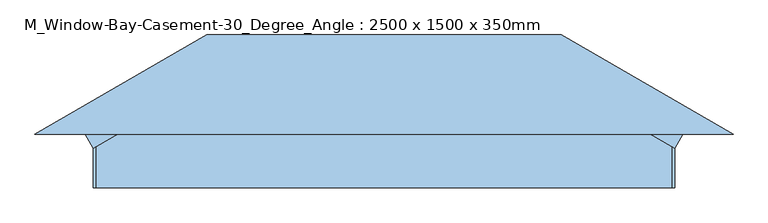
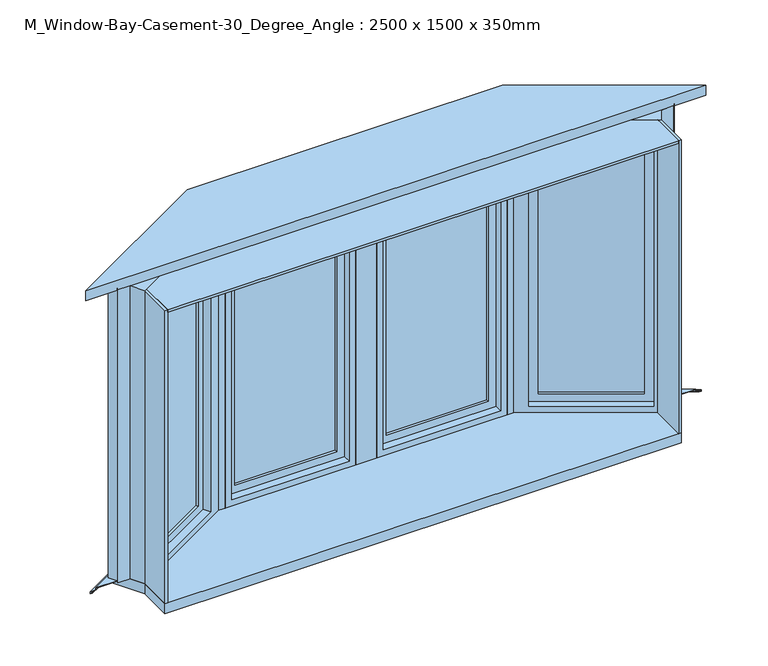
"""IFC4 building model written with IfcOpenShell, lengths in millimetres: window geometry, M_Window-Bay-Casement-30_Degree_Angle : 2500 x 1500 x 350mm."""

from ifc_helpers import new_model, si_unit, frame, origin, place, context, project, spatial, polyline, outline, extrude, faceted_brep, source, transform, mapped, element, save


def m_window_bay_casement_30_degree_angle_2500_x_1500_x_350mm_0714d089(model_context):
    return source(origin(), model_context, "Body", "SolidModel", [
        extrude(outline(polyline([(1224.4331255, 149.925), (1221.2581255, 144.4257387), (835.0107955, 367.4257387), (838.1857955, 372.925), (1224.4331255, 149.925)])), frame((0.0, 0.0, 720.65), z_axis=(0.0, 0.0, 1.0), x_axis=(1.0, 0.0, 0.0)), (0.0, 0.0, 1.0), 1360.3),
        extrude(outline(polyline([(1218.0831255, 138.9264774), (1214.9081255, 133.4272161), (828.6607955, 356.4272161), (831.8357955, 361.9264774), (1218.0831255, 138.9264774)])), frame((0.0, 0.0, 720.65), z_axis=(0.0, 0.0, 1.0), x_axis=(1.0, 0.0, 0.0)), (0.0, 0.0, 1.0), 1360.3),
        extrude(outline(polyline([(1417.45, 57.1500001), (1417.45, -503.15), (-57.15, -503.15), (-57.15, 57.1500001), (1417.45, 57.1500001)]), holes=[polyline([(1360.3, -445.9999999), (1360.3, 0.0), (0.0, 0.0), (0.0, -445.9999999), (1360.3, -445.9999999)])]), frame((1208.5581255, 122.4286934, 720.65), z_axis=(0.49999999999999967, 0.8660254037844388, 0.0), x_axis=(0.0, 0.0, 1.0)), (0.0, 0.0, 1.0), 44.45),
        faceted_brep([(714.9835794, 363.4, 2150.8), (1250.0, 54.5081255, 2150.8), (1284.925, 115.0, 2150.8), (1344.7940905, 115.0, 2150.8), (1344.7940905, 117.0963066, 2150.8), (742.2072174, 465.0, 2150.8), (1258.0514774, 93.8536934, 2138.1), (772.8174436, 374.0036934, 2138.1), (804.5674436, 428.9963066, 2138.1), (1289.8014774, 148.8463066, 2138.1), (1222.5036934, 70.3831255, 2119.05), (770.2652276, 331.4831255, 2119.05), (789.3152276, 364.4786934, 2119.05), (1241.5536934, 103.3786934, 2119.05), (772.8174436, 374.0036934, 663.5), (804.5674436, 428.9963066, 663.5), (770.2652276, 331.4831255, 682.55), (789.3152276, 364.4786934, 682.55), (742.2072174, 465.0, 650.8), (1344.7940905, 117.0963066, 650.8), (1344.7940905, 115.0, 650.8), (1284.925, 115.0, 650.8), (1250.0, 54.5081255, 650.8), (714.9835794, 363.4, 650.8), (1258.0514774, 93.8536934, 663.5), (1289.8014774, 148.8463066, 663.5), (1222.5036934, 70.3831255, 682.55), (1241.5536934, 103.3786934, 682.55)], [[[0, 1, 2, 3, 4, 5]], [[6, 7, 8, 9]], [[10, 11, 12, 13]], [[7, 14, 15, 8]], [[11, 16, 17, 12]], [[18, 19, 20, 21, 22, 23]], [[14, 24, 25, 15]], [[16, 26, 27, 17]], [[22, 21, 2, 1]], [[4, 19, 18, 5], [8, 15, 25, 9]], [[9, 25, 24, 6]], [[6, 24, 14, 7], [12, 17, 27, 13]], [[13, 27, 26, 10]], [[1, 0, 23, 22], [10, 26, 16, 11]], [[5, 18, 23, 0]], [[2, 21, 20, 3]], [[3, 20, 19, 4]]]),
        extrude(outline(polyline([(-1224.4331255, 149.925), (-838.1857955, 372.925), (-835.0107955, 367.4257387), (-1221.2581255, 144.4257387), (-1224.4331255, 149.925)])), frame((0.0, 0.0, 720.65), z_axis=(0.0, 0.0, 1.0), x_axis=(1.0, 0.0, 0.0)), (0.0, 0.0, 1.0), 1360.3),
        extrude(outline(polyline([(-1218.0831255, 138.9264774), (-831.8357955, 361.9264774), (-828.6607955, 356.4272161), (-1214.9081255, 133.4272161), (-1218.0831255, 138.9264774)])), frame((0.0, 0.0, 720.65), z_axis=(0.0, 0.0, 1.0), x_axis=(1.0, 0.0, 0.0)), (0.0, 0.0, 1.0), 1360.3),
        extrude(outline(polyline([(1417.45, -57.1500001), (-57.15, -57.1500001), (-57.15, 503.15), (1417.45, 503.15), (1417.45, -57.1500001)]), holes=[polyline([(1360.3, 445.9999999), (0.0, 445.9999999), (0.0, 0.0), (1360.3, 0.0), (1360.3, 445.9999999)])]), frame((-1208.5581255, 122.4286934, 720.65), z_axis=(-0.49999999999999967, 0.8660254037844388, 0.0), x_axis=(0.0, 0.0, 1.0)), (0.0, 0.0, 1.0), 44.45),
        faceted_brep([(-714.9835794, 363.4, 2150.8), (-742.2072174, 465.0, 2150.8), (-1344.7940905, 117.0963066, 2150.8), (-1344.7940905, 115.0, 2150.8), (-1284.925, 115.0, 2150.8), (-1250.0, 54.5081255, 2150.8), (-1258.0514774, 93.8536934, 2138.1), (-1289.8014774, 148.8463066, 2138.1), (-804.5674436, 428.9963066, 2138.1), (-772.8174436, 374.0036934, 2138.1), (-1222.5036934, 70.3831255, 2119.05), (-1241.5536934, 103.3786934, 2119.05), (-789.3152276, 364.4786934, 2119.05), (-770.2652276, 331.4831255, 2119.05), (-804.5674436, 428.9963066, 663.5), (-772.8174436, 374.0036934, 663.5), (-789.3152276, 364.4786934, 682.55), (-770.2652276, 331.4831255, 682.55), (-742.2072174, 465.0, 650.8), (-714.9835794, 363.4, 650.8), (-1250.0, 54.5081255, 650.8), (-1284.925, 115.0, 650.8), (-1344.7940905, 115.0, 650.8), (-1344.7940905, 117.0963066, 650.8), (-1289.8014774, 148.8463066, 663.5), (-1258.0514774, 93.8536934, 663.5), (-1241.5536934, 103.3786934, 682.55), (-1222.5036934, 70.3831255, 682.55)], [[[0, 1, 2, 3, 4, 5]], [[6, 7, 8, 9]], [[10, 11, 12, 13]], [[9, 8, 14, 15]], [[13, 12, 16, 17]], [[18, 19, 20, 21, 22, 23]], [[15, 14, 24, 25]], [[17, 16, 26, 27]], [[20, 5, 4, 21]], [[2, 1, 18, 23], [8, 7, 24, 14]], [[7, 6, 25, 24]], [[6, 9, 15, 25], [12, 11, 26, 16]], [[11, 10, 27, 26]], [[5, 20, 19, 0], [10, 13, 17, 27]], [[1, 0, 19, 18]], [[4, 3, 22, 21]], [[3, 2, 23, 22]]]),
        faceted_brep([(-755.844462, 515.8, 660.4), (-755.844462, 515.8, 653.0697935), (755.844462, 515.8, 653.0697935), (755.844462, 515.8, 660.4), (-742.232643, 465.0, 663.1486341), (-742.232643, 465.0, 660.4), (742.232643, 465.0, 660.4), (742.232643, 465.0, 663.1486341), (-756.218787, 517.197, 654.4483503), (-756.218787, 517.197, 663.1486341), (756.218787, 517.197, 663.1486341), (756.218787, 517.197, 654.4483503), (759.6217417, 529.897, 652.2089977), (-759.6217417, 529.897, 652.2089977), (759.6217417, 529.897, 643.2668038), (-759.6217417, 529.897, 643.2668038), (-758.5600199, 525.9346, 644.7270038), (-758.5600199, 525.9346, 643.2668038), (758.5600199, 525.9346, 643.2668038), (758.5600199, 525.9346, 644.7270038), (-759.1929694, 528.2968, 650.8662705), (-759.1929694, 528.2968, 644.7270038), (759.1929694, 528.2968, 644.7270038), (759.1929694, 528.2968, 650.8662705), (-1450.0504256, 115.0, 660.4), (-1450.0504256, 115.0, 653.0697935), (1450.0504256, 115.0, 660.4), (1348.4504256, 115.0, 660.4), (-1348.4504256, 115.0, 660.4), (-1348.4504256, 115.0, 663.1486341), (1348.4504256, 115.0, 663.1486341), (1452.8444256, 115.0, 663.1486341), (-1452.8444256, 115.0, 663.1486341), (-1452.8444256, 115.0, 654.4483503), (-1478.2444256, 115.0, 652.2089977), (-1478.2444256, 115.0, 643.2668038), (1478.2444256, 115.0, 643.2668038), (1470.3196257, 115.0, 643.2668038), (-1470.3196257, 115.0, 643.2668038), (-1470.3196257, 115.0, 644.7270038), (1470.3196257, 115.0, 644.7270038), (1475.0440256, 115.0, 644.7270038), (-1475.0440256, 115.0, 644.7270038), (-1475.0440256, 115.0, 650.8662705), (1450.0504256, 115.0, 653.0697935), (1452.8444256, 115.0, 654.4483503), (1478.2444256, 115.0, 652.2089977), (1475.0440256, 115.0, 650.8662705)], [[[0, 1, 2, 3]], [[4, 5, 6, 7]], [[8, 9, 10, 11]], [[8, 11, 12, 13]], [[13, 12, 14, 15]], [[16, 17, 18, 19]], [[20, 21, 22, 23]], [[2, 1, 20, 23]], [[1, 0, 24, 25]], [[0, 3, 26, 27, 6, 5, 28, 24]], [[5, 4, 29, 28]], [[4, 7, 30, 31, 10, 9, 32, 29]], [[9, 8, 33, 32]], [[8, 13, 34, 33]], [[13, 15, 35, 34]], [[15, 14, 36, 37, 18, 17, 38, 35]], [[17, 16, 39, 38]], [[16, 19, 40, 41, 22, 21, 42, 39]], [[21, 20, 43, 42]], [[20, 1, 25, 43]], [[3, 2, 44, 26]], [[7, 6, 27, 30]], [[11, 10, 31, 45]], [[12, 11, 45, 46]], [[14, 12, 46, 36]], [[19, 18, 37, 40]], [[23, 22, 41, 47]], [[2, 23, 47, 44]], [[25, 24, 28, 29, 32, 33, 34, 35, 38, 39, 42, 43]], [[27, 26, 44, 47, 41, 40, 37, 36, 46, 45, 31, 30]]]),
        extrude(outline(polyline([(-1320.9541191, 130.875), (-1348.4504256, 115.0), (-1370.6754256, 153.4948292), (-1343.1791191, 169.3698292), (-1320.9541191, 130.875)])), frame((0.0, 0.0, 663.1486341), z_axis=(0.0, 0.0, 1.0), x_axis=(1.0, 0.0, 0.0)), (0.0, 0.0, 1.0), 1497.2513659),
        extrude(outline(polyline([(1320.9541191, 130.875), (1343.1791191, 169.3698292), (1370.6754256, 153.4948292), (1348.4504256, 115.0), (1320.9541191, 130.875)])), frame((0.0, 0.0, 663.1486341), z_axis=(0.0, 0.0, 1.0), x_axis=(1.0, 0.0, 0.0)), (0.0, 0.0, 1.0), 1497.2513659),
        extrude(outline(polyline([(-714.9835794, 363.4), (714.9835794, 363.4), (1237.3, 61.840474), (1237.3, -115.0), (-1237.3, -115.0), (-1237.3, 61.840474), (-714.9835794, 363.4)])), frame((0.0, 0.0, 2138.1), z_axis=(0.0, 0.0, 1.0), x_axis=(1.0, 0.0, 0.0)), (0.0, 0.0, 1.0), 12.7),
        extrude(outline(polyline([(-1250.0, -115.0), (-1250.0, 54.5081255), (-1237.3, 61.840474), (-1237.3, -115.0), (-1250.0, -115.0)])), frame((0.0, 0.0, 650.8), z_axis=(0.0, 0.0, 1.0), x_axis=(1.0, 0.0, 0.0)), (0.0, 0.0, 1.0), 1500.0),
        extrude(outline(polyline([(1250.0, -115.0), (1237.3, -115.0), (1237.3, 61.840474), (1250.0, 54.5081256), (1250.0, -115.0)])), frame((0.0, 0.0, 650.8), z_axis=(0.0, 0.0, 1.0), x_axis=(1.0, 0.0, 0.0)), (0.0, 0.0, 1.0), 1500.0),
        extrude(outline(polyline([(2138.1, -670.1998305), (663.5, -670.1998305), (663.5, -63.5), (2138.1, -63.5), (2138.1, -670.1998305)]), holes=[polyline([(2080.95, -120.65), (720.65, -120.65), (720.65, -613.0498305), (2080.95, -613.0498305), (2080.95, -120.65)])]), frame((0.0, 401.5, 0.0), z_axis=(0.0, 1.0, 0.0), x_axis=(0.0, 0.0, 1.0)), (0.0, 0.0, 1.0), 44.45),
        extrude(outline(polyline([(2138.1, 63.5), (663.5, 63.5), (663.5, 670.1998305), (2138.1, 670.1998305), (2138.1, 63.5)]), holes=[polyline([(2080.95, 613.0498305), (720.65, 613.0498305), (720.65, 120.65), (2080.95, 120.65), (2080.95, 613.0498305)])]), frame((0.0, 401.5, 0.0), z_axis=(0.0, 1.0, 0.0), x_axis=(0.0, 0.0, 1.0)), (0.0, 0.0, 1.0), 44.45),
        extrude(outline(polyline([(1250.0, -115.0), (-1250.0, -115.0), (-1250.0, 54.5081255), (-1326.2, 186.4903971), (-755.8190363, 515.8), (755.8190363, 515.8), (1326.2, 186.4903971), (1250.0, 54.5081256), (1250.0, -115.0)])), frame((0.0, 0.0, 600.0), z_axis=(0.0, 0.0, 1.0), x_axis=(1.0, 0.0, 0.0)), (0.0, 0.0, 1.0), 50.8),
        faceted_brep([(670.1998305, 401.5, 663.5), (670.1998305, 465.0, 663.5), (63.5, 465.0, 663.5), (63.5, 401.5, 663.5), (651.1498305, 363.4, 682.55), (651.1498305, 401.5, 682.55), (82.55, 401.5, 682.55), (82.55, 363.4, 682.55), (682.8998305, 465.0, 650.8), (682.8998305, 363.4, 650.8), (50.8, 363.4, 650.8), (50.8, 465.0, 650.8), (63.5, 465.0, 2138.1), (63.5, 401.5, 2138.1), (82.55, 401.5, 2119.05), (82.55, 363.4, 2119.05), (50.8, 363.4, 2150.8), (50.8, 465.0, 2150.8), (670.1998305, 465.0, 2138.1), (670.1998305, 401.5, 2138.1), (651.1498305, 401.5, 2119.05), (651.1498305, 363.4, 2119.05), (682.8998305, 363.4, 2150.8), (682.8998305, 465.0, 2150.8)], [[[0, 1, 2, 3]], [[4, 5, 6, 7]], [[8, 9, 10, 11]], [[3, 2, 12, 13]], [[7, 6, 14, 15]], [[11, 10, 16, 17]], [[13, 12, 18, 19]], [[15, 14, 20, 21]], [[17, 16, 22, 23]], [[11, 17, 23, 8], [1, 18, 12, 2]], [[19, 18, 1, 0]], [[3, 13, 19, 0], [5, 20, 14, 6]], [[21, 20, 5, 4]], [[9, 22, 16, 10], [7, 15, 21, 4]], [[23, 22, 9, 8]]]),
        extrude(outline(polyline([(613.0498305, 433.25), (613.0498305, 426.9), (120.65, 426.9), (120.65, 433.25), (613.0498305, 433.25)])), frame((0.0, 0.0, 720.65), z_axis=(0.0, 0.0, 1.0), x_axis=(1.0, 0.0, 0.0)), (0.0, 0.0, 1.0), 1360.3),
        extrude(outline(polyline([(613.0498305, 420.55), (613.0498305, 414.2), (120.65, 414.2), (120.65, 420.55), (613.0498305, 420.55)])), frame((0.0, 0.0, 720.65), z_axis=(0.0, 0.0, 1.0), x_axis=(1.0, 0.0, 0.0)), (0.0, 0.0, 1.0), 1360.3),
        extrude(outline(polyline([(-120.65, 433.25), (-120.65, 426.9), (-613.0498305, 426.9), (-613.0498305, 433.25), (-120.65, 433.25)])), frame((0.0, 0.0, 720.65), z_axis=(0.0, 0.0, 1.0), x_axis=(1.0, 0.0, 0.0)), (0.0, 0.0, 1.0), 1360.3),
        extrude(outline(polyline([(-120.65, 420.55), (-120.65, 414.2), (-613.0498305, 414.2), (-613.0498305, 420.55), (-120.65, 420.55)])), frame((0.0, 0.0, 720.65), z_axis=(0.0, 0.0, 1.0), x_axis=(1.0, 0.0, 0.0)), (0.0, 0.0, 1.0), 1360.3),
        faceted_brep([(-63.5, 401.5, 663.5), (-63.5, 465.0, 663.5), (-670.1998305, 465.0, 663.5), (-670.1998305, 401.5, 663.5), (-82.55, 363.4, 682.55), (-82.55, 401.5, 682.55), (-651.1498305, 401.5, 682.55), (-651.1498305, 363.4, 682.55), (-50.8, 465.0, 650.8), (-50.8, 363.4, 650.8), (-682.8998305, 363.4, 650.8), (-682.8998305, 465.0, 650.8), (-670.1998305, 465.0, 2138.1), (-670.1998305, 401.5, 2138.1), (-651.1498305, 401.5, 2119.05), (-651.1498305, 363.4, 2119.05), (-682.8998305, 363.4, 2150.8), (-682.8998305, 465.0, 2150.8), (-63.5, 465.0, 2138.1), (-63.5, 401.5, 2138.1), (-82.55, 401.5, 2119.05), (-82.55, 363.4, 2119.05), (-50.8, 363.4, 2150.8), (-50.8, 465.0, 2150.8)], [[[0, 1, 2, 3]], [[4, 5, 6, 7]], [[8, 9, 10, 11]], [[3, 2, 12, 13]], [[7, 6, 14, 15]], [[11, 10, 16, 17]], [[13, 12, 18, 19]], [[15, 14, 20, 21]], [[17, 16, 22, 23]], [[11, 17, 23, 8], [1, 18, 12, 2]], [[19, 18, 1, 0]], [[3, 13, 19, 0], [5, 20, 14, 6]], [[21, 20, 5, 4]], [[9, 22, 16, 10], [7, 15, 21, 4]], [[23, 22, 9, 8]]]),
        extrude(outline(polyline([(50.8, 465.0), (50.8, 363.4), (-50.8, 363.4), (-50.8, 465.0), (50.8, 465.0)])), frame((0.0, 0.0, 650.8), z_axis=(0.0, 0.0, 1.0), x_axis=(1.0, 0.0, 0.0)), (0.0, 0.0, 1.0), 1500.0),
        extrude(outline(polyline([(-682.8998305, 465.0), (-682.8998305, 363.4), (-714.9835794, 363.4), (-742.2072173, 465.0), (-682.8998305, 465.0)])), frame((0.0, 0.0, 650.8), z_axis=(0.0, 0.0, 1.0), x_axis=(1.0, 0.0, 0.0)), (0.0, 0.0, 1.0), 1500.0),
        extrude(outline(polyline([(742.2072173, 465.0), (714.9835794, 363.4), (682.8998305, 363.4), (682.8998305, 465.0), (742.2072173, 465.0)])), frame((0.0, 0.0, 650.8), z_axis=(0.0, 0.0, 1.0), x_axis=(1.0, 0.0, 0.0)), (0.0, 0.0, 1.0), 1500.0),
        extrude(outline(polyline([(762.6249458, 541.2), (1500.825, 115.0), (-1500.825, 115.0), (-762.6249458, 541.2), (762.6249458, 541.2)])), frame((0.0, 0.0, 2150.8), z_axis=(0.0, 0.0, 1.0), x_axis=(1.0, 0.0, 0.0)), (0.0, 0.0, 1.0), 50.8),
    ])


if __name__ == "__main__":
    model = new_model("IFC4")
    model_context = context("Model", 3, world=origin())
    ifc_project = project(units=[si_unit("LENGTHUNIT", "METRE", prefix="MILLI")], contexts=[model_context])
    site = spatial("IfcSite", under=ifc_project)
    building = spatial("IfcBuilding", under=site)
    placement = place(None, origin())
    m_window_bay_casement_30_degree_angle_2500_x_1500_x_350mm_shape = m_window_bay_casement_30_degree_angle_2500_x_1500_x_350mm_0714d089(model_context)
    element("IfcWindow", 1, ObjectType="M_Window-Bay-Casement-30_Degree_Angle : 2500 x 1500 x 350mm", at=placement, inside=building, context=model_context, shape_type="MappedRepresentation", body=[
        mapped(m_window_bay_casement_30_degree_angle_2500_x_1500_x_350mm_shape, transform((0.0, 0.0, 0.0), x_axis=(1.0, 0.0, 0.0), y_axis=(0.0, 1.0, 0.0), z_axis=(0.0, 0.0, 1.0))),
    ])
    save(model, "model.ifc")

# Revit data of these elements
# Type "M_Window-Bay-Casement-30_Degree_Angle : 2500 x 1500 x 350mm"
#   Type Mark = "50"
#   Fire Rating = "0.5h"
#   Assembly Code = "B2020100"
#   Analytic Construction = "Double glazing - domestic"
#   Width of Middle Sash = 1365.8 mm
#   Width = 2500 mm
#   Visual Light Transmittance = 0.81
#   Thermal Resistance (R) = 0.319569 (m²·K)/W
#   Solar Heat Gain Coefficient = 0.76
#   Rough Width = 2515 mm
#   Rough Height = 1515 mm
#   Length 2 = 1484.465 mm
#   Length 1 = 516.3 mm
#   Wall Thickness [instance default] = 150 mm
#   Trim Width = 2618.666 mm
#   Trim Height = 1500 mm
#   Height 1 = 1550.8 mm
#   Height = 1500 mm
#   Heat Transfer Coefficient (U) = 3.12929 W/(m²·K)
#   Depth = 350 mm
#   Default Sill Height = 600 mm
#   Angle = 30.00°
#   Muntin Visibility = yes
#   Interior Trim Visibility [instance default] = yes
#   Exterior Trim Visibility [instance default] = yes
#   Muntin Pattern = M_Muntin Pattern_2x2 : M_Muntin Pattern_2x2
#   Interior Trim Material = Wood - Stained
#   Exterior Trim Material = Clad - White
#   Exterior Trim = element 343235
#   Interior Trim = M_Trim-Window-Interior-Flat : Picture Frame
#   Interior Frame Material = Wood - Stained
#   Glass Panel Material = Glass
#   Exterior Frame Material = Clad - White
#   Wall Closure = (empty or 0)
# Element 1 (IfcWindow, "M_Window-Bay-Casement-30_Degree_Angle : 2500 x 1500 x 350mm")
#   Wall Thickness = 230 mm
#   Materials on its faces: "Clad - White", "Wood - Stained", "Glass"
# Materials
#   "Wood - Stained": class "Wood", colour RGB 227 170 128, transparency 0, Cost = 0
#   "Clad - White": class "Wood", colour RGB 242 242 238, transparency 0, Cost = 0
#   "Glass": class "Glass", colour RGB 0 128 192, transparency 0.9, Description = "Soda Lime Glass", Cost = 0
